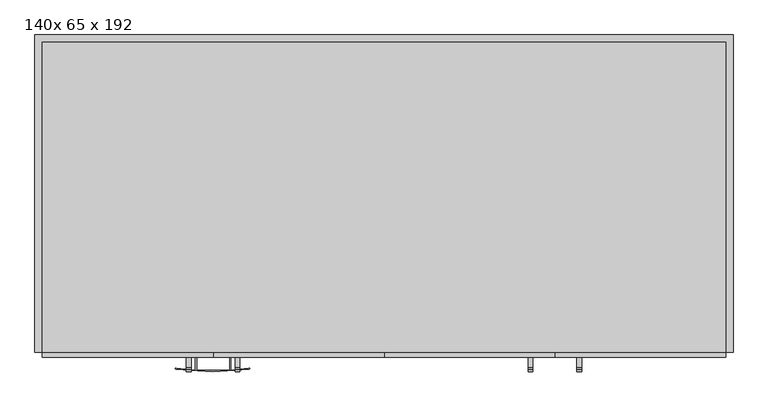
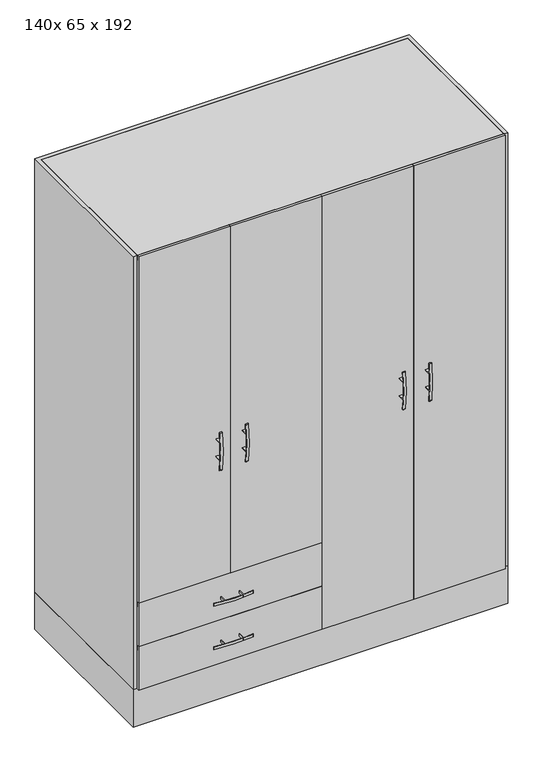
"""IFC4 building model written with IfcOpenShell, lengths in millimetres: furniture geometry, Wardrobe_-_Guarda_roupa_simples_18250 : 140x 65 x 192."""

from ifc_helpers import new_model, si_unit, point, frame, frame_2d, origin, origin_with_axes, place, context, project, spatial, polyline, circle_curve, trimmed, segment, composite_curve, outline, extrude, source, transform, mapped, element, save


def furniture_140x_65_x_192_42ee9c7a(model_context):
    return source(origin(), model_context, "Body", "SweptSolid", [
        extrude(outline(composite_curve([segment(polyline([(-316.25, -660.0), (-313.75, -660.0), (-313.75, -686.1172605)]), True, "CONTINUOUS"), segment(trimmed(circle_curve(frame_2d((-351.25, -178.3072148)), 509.1927852), [point((-313.75, -686.1172605))], [point((-276.6164308, -682.0006958))], True, "CARTESIAN"), True, "CONTINUOUS"), segment(trimmed(circle_curve(frame_2d((-276.6164308, -683.2642755)), 1.2635797), [point((-276.6164308, -682.0006958))], [point((-276.2508973, -684.4738287))], False, "CARTESIAN"), True, "CONTINUOUS"), segment(trimmed(circle_curve(frame_2d((-351.25, -178.3072148)), 511.6927852), [point((-276.2508973, -684.4738287))], [point((-426.2491027, -684.4738287))], False, "CARTESIAN"), True, "CONTINUOUS"), segment(trimmed(circle_curve(frame_2d((-425.8835692, -683.2642755)), 1.2635797), [point((-426.2491027, -684.4738287))], [point((-425.8835692, -682.0006958))], False, "CARTESIAN"), True, "CONTINUOUS"), segment(trimmed(circle_curve(frame_2d((-351.25, -178.3072148)), 509.1927852), [point((-425.8835692, -682.0006958))], [point((-386.25, -686.2956915))], True, "CARTESIAN"), True, "CONTINUOUS"), segment(polyline([(-386.25, -686.2956915), (-386.25, -660.0), (-383.75, -660.0), (-383.75, -686.4617607)]), True, "CONTINUOUS"), segment(trimmed(circle_curve(frame_2d((-351.25, -178.3072148)), 509.1927852), [point((-383.75, -686.4617607))], [point((-316.25, -686.2956915))], True, "CARTESIAN"), True, "CONTINUOUS"), segment(polyline([(-316.25, -686.2956915), (-316.25, -660.0)]), True, "CONTINUOUS")], self_intersect=False)), frame((0.0, 0.0, 232.5), z_axis=(0.0, 0.0, 1.0), x_axis=(1.0, 0.0, 0.0)), (0.0, 0.0, 1.0), 10.0),
        extrude(outline(composite_curve([segment(polyline([(-660.0, 1061.25), (-660.0, 1058.75), (-686.2956915, 1058.75)]), True, "CONTINUOUS"), segment(trimmed(circle_curve(frame_2d((-178.3072148, 1023.75)), 509.1927852), [point((-686.2956915, 1058.75))], [point((-686.4617607, 991.25))], True, "CARTESIAN"), True, "CONTINUOUS"), segment(polyline([(-686.4617607, 991.25), (-660.0, 991.25), (-660.0, 988.75), (-686.2956915, 988.75)]), True, "CONTINUOUS"), segment(trimmed(circle_curve(frame_2d((-178.3072148, 1023.75)), 509.1927852), [point((-686.2956915, 988.75))], [point((-682.0006958, 949.1164308))], True, "CARTESIAN"), True, "CONTINUOUS"), segment(trimmed(circle_curve(frame_2d((-683.2642755, 949.1164308)), 1.2635797), [point((-682.0006958, 949.1164308))], [point((-684.4738287, 948.7508973))], False, "CARTESIAN"), True, "CONTINUOUS"), segment(trimmed(circle_curve(frame_2d((-178.3072148, 1023.75)), 511.6927852), [point((-684.4738287, 948.7508973))], [point((-684.4738287, 1098.7491027))], False, "CARTESIAN"), True, "CONTINUOUS"), segment(trimmed(circle_curve(frame_2d((-683.2642755, 1098.3835692)), 1.2635797), [point((-684.4738287, 1098.7491027))], [point((-682.0006958, 1098.3835692))], False, "CARTESIAN"), True, "CONTINUOUS"), segment(trimmed(circle_curve(frame_2d((-178.3072148, 1023.75)), 509.1927852), [point((-682.0006958, 1098.3835692))], [point((-686.1172605, 1061.25))], True, "CARTESIAN"), True, "CONTINUOUS"), segment(polyline([(-686.1172605, 1061.25), (-660.0, 1061.25)]), True, "CONTINUOUS")], self_intersect=False)), frame((395.0, 0.0, 0.0), z_axis=(1.0, 0.0, 0.0), x_axis=(0.0, 1.0, 0.0)), (0.0, 0.0, 1.0), 10.0),
        extrude(outline(composite_curve([segment(polyline([(-660.0, 1061.25), (-660.0, 1058.75), (-686.2956915, 1058.75)]), True, "CONTINUOUS"), segment(trimmed(circle_curve(frame_2d((-178.3072148, 1023.75)), 509.1927852), [point((-686.2956915, 1058.75))], [point((-686.4617607, 991.25))], True, "CARTESIAN"), True, "CONTINUOUS"), segment(polyline([(-686.4617607, 991.25), (-660.0, 991.25), (-660.0, 988.75), (-686.2956915, 988.75)]), True, "CONTINUOUS"), segment(trimmed(circle_curve(frame_2d((-178.3072148, 1023.75)), 509.1927852), [point((-686.2956915, 988.75))], [point((-682.0006958, 949.1164308))], True, "CARTESIAN"), True, "CONTINUOUS"), segment(trimmed(circle_curve(frame_2d((-683.2642755, 949.1164308)), 1.2635797), [point((-682.0006958, 949.1164308))], [point((-684.4738287, 948.7508973))], False, "CARTESIAN"), True, "CONTINUOUS"), segment(trimmed(circle_curve(frame_2d((-178.3072148, 1023.75)), 511.6927852), [point((-684.4738287, 948.7508973))], [point((-684.4738287, 1098.7491027))], False, "CARTESIAN"), True, "CONTINUOUS"), segment(trimmed(circle_curve(frame_2d((-683.2642755, 1098.3835692)), 1.2635797), [point((-684.4738287, 1098.7491027))], [point((-682.0006958, 1098.3835692))], False, "CARTESIAN"), True, "CONTINUOUS"), segment(trimmed(circle_curve(frame_2d((-178.3072148, 1023.75)), 509.1927852), [point((-682.0006958, 1098.3835692))], [point((-686.1172605, 1061.25))], True, "CARTESIAN"), True, "CONTINUOUS"), segment(polyline([(-686.1172605, 1061.25), (-660.0, 1061.25)]), True, "CONTINUOUS")], self_intersect=False)), frame((295.0, 0.0, 0.0), z_axis=(1.0, 0.0, 0.0), x_axis=(0.0, 1.0, 0.0)), (0.0, 0.0, 1.0), 10.0),
        extrude(outline(composite_curve([segment(polyline([(-660.0, 1061.25), (-660.0, 1058.75), (-686.2956915, 1058.75)]), True, "CONTINUOUS"), segment(trimmed(circle_curve(frame_2d((-178.3072148, 1023.75)), 509.1927852), [point((-686.2956915, 1058.75))], [point((-686.4617607, 991.25))], True, "CARTESIAN"), True, "CONTINUOUS"), segment(polyline([(-686.4617607, 991.25), (-660.0, 991.25), (-660.0, 988.75), (-686.2956915, 988.75)]), True, "CONTINUOUS"), segment(trimmed(circle_curve(frame_2d((-178.3072148, 1023.75)), 509.1927852), [point((-686.2956915, 988.75))], [point((-682.0006958, 949.1164308))], True, "CARTESIAN"), True, "CONTINUOUS"), segment(trimmed(circle_curve(frame_2d((-683.2642755, 949.1164308)), 1.2635797), [point((-682.0006958, 949.1164308))], [point((-684.4738287, 948.7508973))], False, "CARTESIAN"), True, "CONTINUOUS"), segment(trimmed(circle_curve(frame_2d((-178.3072148, 1023.75)), 511.6927852), [point((-684.4738287, 948.7508973))], [point((-684.4738287, 1098.7491027))], False, "CARTESIAN"), True, "CONTINUOUS"), segment(trimmed(circle_curve(frame_2d((-683.2642755, 1098.3835692)), 1.2635797), [point((-684.4738287, 1098.7491027))], [point((-682.0006958, 1098.3835692))], False, "CARTESIAN"), True, "CONTINUOUS"), segment(trimmed(circle_curve(frame_2d((-178.3072148, 1023.75)), 509.1927852), [point((-682.0006958, 1098.3835692))], [point((-686.1172605, 1061.25))], True, "CARTESIAN"), True, "CONTINUOUS"), segment(polyline([(-686.1172605, 1061.25), (-660.0, 1061.25)]), True, "CONTINUOUS")], self_intersect=False)), frame((-305.0, 0.0, 0.0), z_axis=(1.0, 0.0, 0.0), x_axis=(0.0, 1.0, 0.0)), (0.0, 0.0, 1.0), 10.0),
        extrude(outline(composite_curve([segment(polyline([(-316.25, -660.0), (-313.75, -660.0), (-313.75, -686.1172605)]), True, "CONTINUOUS"), segment(trimmed(circle_curve(frame_2d((-351.25, -178.3072148)), 509.1927852), [point((-313.75, -686.1172605))], [point((-276.6164308, -682.0006958))], True, "CARTESIAN"), True, "CONTINUOUS"), segment(trimmed(circle_curve(frame_2d((-276.6164308, -683.2642755)), 1.2635797), [point((-276.6164308, -682.0006958))], [point((-276.2508973, -684.4738287))], False, "CARTESIAN"), True, "CONTINUOUS"), segment(trimmed(circle_curve(frame_2d((-351.25, -178.3072148)), 511.6927852), [point((-276.2508973, -684.4738287))], [point((-426.2491027, -684.4738287))], False, "CARTESIAN"), True, "CONTINUOUS"), segment(trimmed(circle_curve(frame_2d((-425.8835692, -683.2642755)), 1.2635797), [point((-426.2491027, -684.4738287))], [point((-425.8835692, -682.0006958))], False, "CARTESIAN"), True, "CONTINUOUS"), segment(trimmed(circle_curve(frame_2d((-351.25, -178.3072148)), 509.1927852), [point((-425.8835692, -682.0006958))], [point((-386.25, -686.2956915))], True, "CARTESIAN"), True, "CONTINUOUS"), segment(polyline([(-386.25, -686.2956915), (-386.25, -660.0), (-383.75, -660.0), (-383.75, -686.4617607)]), True, "CONTINUOUS"), segment(trimmed(circle_curve(frame_2d((-351.25, -178.3072148)), 509.1927852), [point((-383.75, -686.4617607))], [point((-316.25, -686.2956915))], True, "CARTESIAN"), True, "CONTINUOUS"), segment(polyline([(-316.25, -686.2956915), (-316.25, -660.0)]), True, "CONTINUOUS")], self_intersect=False)), frame((0.0, 0.0, 407.5), z_axis=(0.0, 0.0, 1.0), x_axis=(1.0, 0.0, 0.0)), (0.0, 0.0, 1.0), 10.0),
        extrude(outline(composite_curve([segment(polyline([(-660.0, 1061.25), (-660.0, 1058.75), (-686.2956915, 1058.75)]), True, "CONTINUOUS"), segment(trimmed(circle_curve(frame_2d((-178.3072148, 1023.75)), 509.1927852), [point((-686.2956915, 1058.75))], [point((-686.4617607, 991.25))], True, "CARTESIAN"), True, "CONTINUOUS"), segment(polyline([(-686.4617607, 991.25), (-660.0, 991.25), (-660.0, 988.75), (-686.2956915, 988.75)]), True, "CONTINUOUS"), segment(trimmed(circle_curve(frame_2d((-178.3072148, 1023.75)), 509.1927852), [point((-686.2956915, 988.75))], [point((-682.0006958, 949.1164308))], True, "CARTESIAN"), True, "CONTINUOUS"), segment(trimmed(circle_curve(frame_2d((-683.2642755, 949.1164308)), 1.2635797), [point((-682.0006958, 949.1164308))], [point((-684.4738287, 948.7508973))], False, "CARTESIAN"), True, "CONTINUOUS"), segment(trimmed(circle_curve(frame_2d((-178.3072148, 1023.75)), 511.6927852), [point((-684.4738287, 948.7508973))], [point((-684.4738287, 1098.7491027))], False, "CARTESIAN"), True, "CONTINUOUS"), segment(trimmed(circle_curve(frame_2d((-683.2642755, 1098.3835692)), 1.2635797), [point((-684.4738287, 1098.7491027))], [point((-682.0006958, 1098.3835692))], False, "CARTESIAN"), True, "CONTINUOUS"), segment(trimmed(circle_curve(frame_2d((-178.3072148, 1023.75)), 509.1927852), [point((-682.0006958, 1098.3835692))], [point((-686.1172605, 1061.25))], True, "CARTESIAN"), True, "CONTINUOUS"), segment(polyline([(-686.1172605, 1061.25), (-660.0, 1061.25)]), True, "CONTINUOUS")], self_intersect=False)), frame((-405.0, 0.0, 0.0), z_axis=(1.0, 0.0, 0.0), x_axis=(0.0, 1.0, 0.0)), (0.0, 0.0, 1.0), 10.0),
        extrude(outline(polyline([(10.0, -650.0), (0.0, -650.0), (0.0, -15.0), (10.0, -15.0), (10.0, -650.0)])), frame((0.0, 0.0, 150.0), z_axis=(0.0, 0.0, 1.0), x_axis=(1.0, 0.0, 0.0)), (0.0, 0.0, 1.0), 350.0),
        extrude(outline(polyline([(715.0, -650.0), (-715.0, -650.0), (-715.0, 0.0), (715.0, 0.0), (715.0, -650.0)])), origin_with_axes(), (0.0, 0.0, 1.0), 150.0),
        extrude(outline(polyline([(0.0, -650.0), (-700.0, -650.0), (-700.0, -15.0), (0.0, -15.0), (0.0, -650.0)])), frame((0.0, 0.0, 305.0), z_axis=(0.0, 0.0, 1.0), x_axis=(1.0, 0.0, 0.0)), (0.0, 0.0, 1.0), 20.0),
        extrude(outline(polyline([(700.0, -650.0), (-700.0, -650.0), (-700.0, -15.0), (700.0, -15.0), (700.0, -650.0)])), frame((0.0, 0.0, 1880.0), z_axis=(0.0, 0.0, 1.0), x_axis=(1.0, 0.0, 0.0)), (0.0, 0.0, 1.0), 20.0),
        extrude(outline(polyline([(0.0, -650.0), (-700.0, -650.0), (-700.0, -15.0), (0.0, -15.0), (0.0, -650.0)])), frame((0.0, 0.0, 480.0), z_axis=(0.0, 0.0, 1.0), x_axis=(1.0, 0.0, 0.0)), (0.0, 0.0, 1.0), 20.0),
        extrude(outline(polyline([(0.0, -660.0), (-700.0, -660.0), (-700.0, -650.0), (0.0, -650.0), (0.0, -660.0)])), frame((0.0, 0.0, 150.0), z_axis=(0.0, 0.0, 1.0), x_axis=(1.0, 0.0, 0.0)), (0.0, 0.0, 1.0), 175.0),
        extrude(outline(polyline([(0.0, -660.0), (-700.0, -660.0), (-700.0, -650.0), (0.0, -650.0), (0.0, -660.0)])), frame((0.0, 0.0, 325.0), z_axis=(0.0, 0.0, 1.0), x_axis=(1.0, 0.0, 0.0)), (0.0, 0.0, 1.0), 175.0),
        extrude(outline(polyline([(-350.0, -660.0), (-700.0, -660.0), (-700.0, -650.0), (-350.0, -650.0), (-350.0, -660.0)])), frame((0.0, 0.0, 500.0), z_axis=(0.0, 0.0, 1.0), x_axis=(1.0, 0.0, 0.0)), (0.0, 0.0, 1.0), 1400.0),
        extrude(outline(polyline([(0.0, -660.0), (-350.0, -660.0), (-350.0, -650.0), (0.0, -650.0), (0.0, -660.0)])), frame((0.0, 0.0, 500.0), z_axis=(0.0, 0.0, 1.0), x_axis=(1.0, 0.0, 0.0)), (0.0, 0.0, 1.0), 1400.0),
        extrude(outline(polyline([(350.0, -660.0), (0.0, -660.0), (0.0, -650.0), (350.0, -650.0), (350.0, -660.0)])), frame((0.0, 0.0, 150.0), z_axis=(0.0, 0.0, 1.0), x_axis=(1.0, 0.0, 0.0)), (0.0, 0.0, 1.0), 1750.0),
        extrude(outline(polyline([(700.0, -660.0), (350.0, -660.0), (350.0, -650.0), (700.0, -650.0), (700.0, -660.0)])), frame((0.0, 0.0, 150.0), z_axis=(0.0, 0.0, 1.0), x_axis=(1.0, 0.0, 0.0)), (0.0, 0.0, 1.0), 1750.0),
        extrude(outline(polyline([(-700.0, -650.0), (-715.0, -650.0), (-715.0, 0.0), (715.0, 0.0), (715.0, -650.0), (700.0, -650.0), (700.0, -15.0), (-700.0, -15.0), (-700.0, -650.0)])), frame((0.0, 0.0, 150.0), z_axis=(0.0, 0.0, 1.0), x_axis=(1.0, 0.0, 0.0)), (0.0, 0.0, 1.0), 1750.0),
    ])


if __name__ == "__main__":
    model = new_model("IFC4")
    model_context = context("Model", 3, world=origin())
    ifc_project = project(units=[si_unit("LENGTHUNIT", "METRE", prefix="MILLI")], contexts=[model_context])
    site = spatial("IfcSite", under=ifc_project)
    building = spatial("IfcBuilding", under=site)
    placement = place(None, origin())
    furniture_140x_65_x_192_shape = furniture_140x_65_x_192_42ee9c7a(model_context)
    element("IfcFurniture", 1, ObjectType="Wardrobe_-_Guarda_roupa_simples_18250 : 140x 65 x 192", at=placement, inside=building, context=model_context, shape_type="MappedRepresentation", body=[
        mapped(furniture_140x_65_x_192_shape, transform((0.0, 0.0, 0.0), x_axis=(1.0, 0.0, 0.0), y_axis=(0.0, 1.0, 0.0), z_axis=(0.0, 0.0, 1.0))),
    ])
    save(model, "model.ifc")

# Revit data of these elements
# Type "Wardrobe_-_Guarda_roupa_simples_18250 : 140x 65 x 192"
#   Profundidade = 0.65 m
#   Largura = 1.4 m
#   Altura = 1.9 m
#   Puxador = Handle
#   Painéis = wood brown
#   Default Elevation = 0
# Element 1 (IfcFurniture, "Wardrobe_-_Guarda_roupa_simples_18250 : 140x 65 x 192")
#   Materials on its faces: "wood brown", "Handle"
# Materials
#   "Handle": class "Não atribuído", colour RGB 247 247 247, transparency 0, Cost = 0
#   "wood brown": class "Wood", colour RGB 80 39 12, transparency 0, Cost = 0
